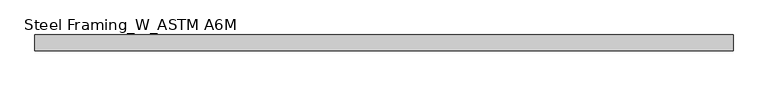
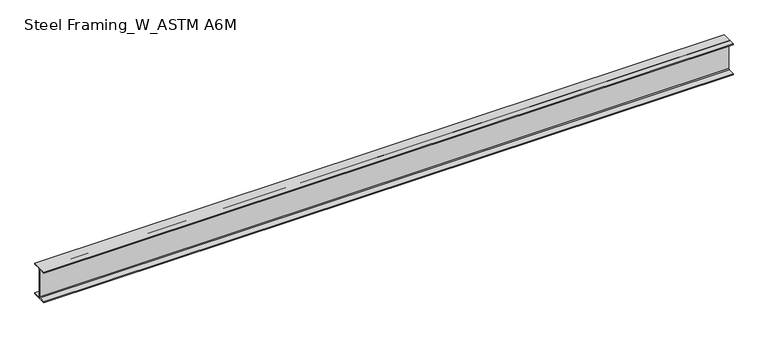
"""IFC4 building model written with IfcOpenShell, lengths in millimetres: beam geometry, Steel Framing_W_ASTM A6M : H_SB_AR_S02_W360x51_RG1."""

import ifcopenshell
import ifcopenshell.guid

model = None  # the IFC model being written
_history = None  # IfcOwnerHistory: only IFC2X3 demands one
_inside = {}  # id of a spatial element -> (the spatial element, [elements in it])
_under = {}  # id of a project, library or spatial element -> (it, [spatial elements below it])
_declared = {}  # id of a project -> (the project, [libraries it declares])
_typed = {}  # id of a type object -> (the type object, [elements of that type])
_made_of = {}  # id of a material, layer set ... -> (it, [elements and type objects made of it])


def new_model(schema):
    """Start an empty IFC model of exactly this schema.

    Asked for "IFC4X3", IfcOpenShell would pick the latest addendum, in which some entities
    have other attributes; the version numbers below select the first issue.
    IFC2X3 requires an IfcOwnerHistory on every rooted entity: one is made here for all.
    """
    global model, _history
    if schema == "IFC4X3":
        model = ifcopenshell.file(schema_version=(4, 3, 0, 0))
    else:
        model = ifcopenshell.file(schema=schema)
    _inside.clear()
    _under.clear()
    _declared.clear()
    _typed.clear()
    _made_of.clear()
    _history = None
    if model.schema == "IFC2X3":
        org = make("IfcOrganization", Name="unknown")
        user = make(
            "IfcPersonAndOrganization",
            ThePerson=make("IfcPerson", FamilyName="unknown"),
            TheOrganization=org,
        )
        app = make(
            "IfcApplication",
            ApplicationDeveloper=org,
            Version="unknown",
            ApplicationFullName="unknown",
            ApplicationIdentifier="unknown",
        )
        _history = make(
            "IfcOwnerHistory",
            OwningUser=user,
            OwningApplication=app,
            ChangeAction="ADDED",
            CreationDate=0,
        )
    return model


def make(cls, **values):
    """One entity of the class cls with the attributes given. An attribute that is None is left unset."""
    return model.create_entity(
        cls, **{name: value for name, value in values.items() if value is not None}
    )


def rooted(cls, **values):
    """An entity with a GlobalId (a new one), such as an element, a storey or a relation."""
    return make(cls, GlobalId=ifcopenshell.guid.new(), OwnerHistory=_history, **values)


def si_unit(unit_type, name, prefix=None):
    """IfcSIUnit, for example si_unit("LENGTHUNIT", "METRE", prefix="MILLI")."""
    return make("IfcSIUnit", UnitType=unit_type, Prefix=prefix, Name=name)


def assignment(units):
    """IfcUnitAssignment: the units of a project."""
    return None if units is None else make("IfcUnitAssignment", Units=units)


def point(xyz):
    """IfcCartesianPoint."""
    return None if xyz is None else make("IfcCartesianPoint", Coordinates=xyz)


def direction(xyz):
    """IfcDirection."""
    return None if xyz is None else make("IfcDirection", DirectionRatios=xyz)


def frame(location, z_axis=None, x_axis=None):
    """IfcAxis2Placement3D, a coordinate frame: its origin and axes. An axis left out is left unset."""
    return make(
        "IfcAxis2Placement3D",
        Location=point(location),
        Axis=direction(z_axis),
        RefDirection=direction(x_axis),
    )


def frame_2d(location, x_axis=None):
    """IfcAxis2Placement2D, a coordinate frame in the plane: its origin and x axis."""
    return make(
        "IfcAxis2Placement2D", Location=point(location), RefDirection=direction(x_axis)
    )


def origin():
    """The frame at (0, 0, 0) with its axes left unset."""
    return frame((0.0, 0.0, 0.0))


def place(relative_to, where):
    """IfcLocalPlacement: puts the frame where relative to a parent placement (None: the world)."""
    return make(
        "IfcLocalPlacement", PlacementRelTo=relative_to, RelativePlacement=where
    )


def context(
    kind, dimensions, precision=None, world=None, true_north=None, identifier=None
):
    """IfcGeometricRepresentationContext, for example the 3D "Model" context."""
    return make(
        "IfcGeometricRepresentationContext",
        ContextIdentifier=identifier,
        ContextType=kind,
        CoordinateSpaceDimension=dimensions,
        Precision=precision,
        WorldCoordinateSystem=world,
        TrueNorth=true_north,
    )


def project(units=None, contexts=None):
    """IfcProject with its units and contexts."""
    return rooted(
        "IfcProject",
        Name="project",
        RepresentationContexts=contexts,
        UnitsInContext=assignment(units),
    )


def spatial(cls, under=None, at=None, **own):
    """A site, building, storey or space (cls), placed at a placement, below another one or the project."""
    s = rooted(cls, ObjectPlacement=at, **own)
    if under is not None:
        _under.setdefault(under.id(), (under, []))[1].append(s)
    return s


def polyline(points):
    """IfcPolyline through the points."""
    return make("IfcPolyline", Points=[point(p) for p in points])


def circle_curve(where, radius):
    """IfcCircle in the frame where."""
    return make("IfcCircle", Position=where, Radius=radius)


def trimmed(basis, trim1, trim2, sense, master):
    """IfcTrimmedCurve: the piece of a basis curve between two trims."""
    return make(
        "IfcTrimmedCurve",
        BasisCurve=basis,
        Trim1=trim1,
        Trim2=trim2,
        SenseAgreement=sense,
        MasterRepresentation=master,
    )


def segment(curve, same_sense, transition):
    """IfcCompositeCurveSegment."""
    return make(
        "IfcCompositeCurveSegment",
        Transition=transition,
        SameSense=same_sense,
        ParentCurve=curve,
    )


def composite_curve(segments, self_intersect=None):
    """IfcCompositeCurve: segments joined end to end."""
    return make("IfcCompositeCurve", Segments=segments, SelfIntersect=self_intersect)


def outline(outer, holes=None, kind="AREA"):
    """IfcArbitraryClosedProfileDef: a profile drawn as a closed curve; with holes, ...WithVoids."""
    if holes is None:
        return make("IfcArbitraryClosedProfileDef", ProfileType=kind, OuterCurve=outer)
    return make(
        "IfcArbitraryProfileDefWithVoids",
        ProfileType=kind,
        OuterCurve=outer,
        InnerCurves=holes,
    )


def extrude(swept, where, along, depth):
    """IfcExtrudedAreaSolid: the profile swept, set in the frame where, extruded along a direction by depth."""
    return make(
        "IfcExtrudedAreaSolid",
        SweptArea=swept,
        Position=where,
        ExtrudedDirection=direction(along),
        Depth=depth,
    )


def shape(context_of_items, identifier, shape_type, items):
    """IfcShapeRepresentation: the items that make up one representation, for example the "Body"."""
    return make(
        "IfcShapeRepresentation",
        ContextOfItems=context_of_items,
        RepresentationIdentifier=identifier,
        RepresentationType=shape_type,
        Items=items,
    )


def source(mapping_origin, context_of_items, identifier, shape_type, items):
    """IfcRepresentationMap: a shape defined once, which mapped items show again and again."""
    return make(
        "IfcRepresentationMap",
        MappingOrigin=mapping_origin,
        MappedRepresentation=shape(context_of_items, identifier, shape_type, items),
    )


def transform(
    local_origin,
    x_axis=None,
    y_axis=None,
    z_axis=None,
    scale=None,
    scale2=None,
    scale3=None,
    uniform=True,
):
    """IfcCartesianTransformationOperator3D, or its non-uniform kind. x_axis, y_axis, z_axis: its Axis1, 2, 3."""
    if uniform:
        return make(
            "IfcCartesianTransformationOperator3D",
            Axis1=direction(x_axis),
            Axis2=direction(y_axis),
            LocalOrigin=point(local_origin),
            Scale=scale,
            Axis3=direction(z_axis),
        )
    return make(
        "IfcCartesianTransformationOperator3DnonUniform",
        Axis1=direction(x_axis),
        Axis2=direction(y_axis),
        LocalOrigin=point(local_origin),
        Scale=scale,
        Axis3=direction(z_axis),
        Scale2=scale2,
        Scale3=scale3,
    )


def mapped(mapping_source, mapping_target):
    """IfcMappedItem: shows the shape of a source again, moved by a transform."""
    return make(
        "IfcMappedItem", MappingSource=mapping_source, MappingTarget=mapping_target
    )


def made_of(thing, what):
    """Note that an element or type object is made of a material, layer set ...; save() writes the relation."""
    if what is not None:
        _made_of.setdefault(what.id(), (what, []))[1].append(thing)
    return thing


def element(
    cls,
    number,
    at=None,
    inside=None,
    cuts=None,
    type_object=None,
    material=None,
    context=None,
    identifier="Body",
    shape_type=None,
    held_by="IfcProductDefinitionShape",
    body=None,
    shapes=None,
    **own,
):
    """One element of the class cls, such as IfcWall. Its Tag is "e" and its number.

    at: its placement. inside: the storey or other place that contains it. cuts: it is an
    opening in that element (IfcRelVoidsElement). A single representation is given by context,
    identifier, shape_type and body (its items); several are given by shapes. held_by: the class
    of the entity that holds the representations. save() writes the other relations.
    """
    e = rooted(cls, Tag="e%d" % number, ObjectPlacement=at, **own)
    if body is not None:
        shapes = [shape(context, identifier, shape_type, body)]
    if shapes is not None:
        e.Representation = make(held_by, Representations=shapes)
    if inside is not None:
        _inside.setdefault(inside.id(), (inside, []))[1].append(e)
    if cuts is not None:
        rooted(
            "IfcRelVoidsElement", RelatingBuildingElement=cuts, RelatedOpeningElement=e
        )
    if type_object is not None:
        _typed.setdefault(type_object.id(), (type_object, []))[1].append(e)
    return made_of(e, material)


def aggregate(whole, parts):
    """IfcRelAggregates: a whole, such as a stair, and the parts it consists of."""
    return rooted("IfcRelAggregates", RelatingObject=whole, RelatedObjects=parts)


def save(model, path):
    """Write the relations noted so far, then the file.

    IfcRelAggregates (storeys below a building ...), IfcRelContainedInSpatialStructure (elements
    in a storey), IfcRelDefinesByType, IfcRelAssociatesMaterial and IfcRelDeclares: one each for
    every whole, place, type object, material and project.
    """
    for whole, parts in _under.values():
        aggregate(whole, parts)
    for where, things in _inside.values():
        rooted(
            "IfcRelContainedInSpatialStructure",
            RelatedElements=things,
            RelatingStructure=where,
        )
    for kind, things in _typed.values():
        rooted("IfcRelDefinesByType", RelatedObjects=things, RelatingType=kind)
    for what, things in _made_of.values():
        rooted("IfcRelAssociatesMaterial", RelatedObjects=things, RelatingMaterial=what)
    for by, libraries in _declared.values():
        rooted("IfcRelDeclares", RelatingContext=by, RelatedDefinitions=libraries)
    model.write(path)


def steel_framing_w_astm_a6m_20e71bf1(model_context):
    return source(origin(), model_context, "Body", "SweptSolid", [
        extrude(outline(composite_curve([segment(polyline([(85.5, -166.4), (85.5, -178.0), (-85.5, -178.0), (-85.5, -166.4), (-13.72, -166.4)]), True, "CONTINUOUS"), segment(trimmed(circle_curve(frame_2d((-13.72, -156.3)), 10.1), [point((-13.72, -166.4))], [point((-3.62, -156.3))], True, "CARTESIAN"), True, "CONTINUOUS"), segment(polyline([(-3.62, -156.3), (-3.62, 156.3)]), True, "CONTINUOUS"), segment(trimmed(circle_curve(frame_2d((-13.72, 156.3)), 10.1), [point((-3.62, 156.3))], [point((-13.72, 166.4))], True, "CARTESIAN"), True, "CONTINUOUS"), segment(polyline([(-13.72, 166.4), (-85.5, 166.4), (-85.5, 178.0), (85.5, 178.0), (85.5, 166.4), (13.72, 166.4)]), True, "CONTINUOUS"), segment(trimmed(circle_curve(frame_2d((13.72, 156.3)), 10.1), [point((13.72, 166.4))], [point((3.62, 156.3))], True, "CARTESIAN"), True, "CONTINUOUS"), segment(polyline([(3.62, 156.3), (3.62, -156.3)]), True, "CONTINUOUS"), segment(trimmed(circle_curve(frame_2d((13.72, -156.3)), 10.1), [point((3.62, -156.3))], [point((13.72, -166.4))], True, "CARTESIAN"), True, "CONTINUOUS"), segment(polyline([(13.72, -166.4), (85.5, -166.4)]), True, "CONTINUOUS")], self_intersect=False)), frame((-3748.7, 0.0, 0.0), z_axis=(1.0, 0.0, 0.0), x_axis=(0.0, 1.0, 0.0)), (0.0, 0.0, 1.0), 7566.7),
    ])


if __name__ == "__main__":
    model = new_model("IFC4")
    model_context = context("Model", 3, world=origin())
    ifc_project = project(units=[si_unit("LENGTHUNIT", "METRE", prefix="MILLI")], contexts=[model_context])
    site = spatial("IfcSite", under=ifc_project)
    building = spatial("IfcBuilding", under=site)
    placement = place(None, origin())
    steel_framing_w_astm_a6m_shape = steel_framing_w_astm_a6m_20e71bf1(model_context)
    element("IfcBeam", 1, ObjectType="Steel Framing_W_ASTM A6M : H_SB_AR_S02_W360x51_RG1", at=placement, inside=building, context=model_context, shape_type="MappedRepresentation", body=[
        mapped(steel_framing_w_astm_a6m_shape, transform((0.0, 0.0, 0.0), x_axis=(1.0, 0.0, 0.0), y_axis=(0.0, 1.0, 0.0), z_axis=(0.0, 0.0, 1.0))),
    ])
    save(model, "model.ifc")

# Revit data of these elements
# Type "Steel Framing_W_ASTM A6M : H_SB_AR_S02_W360x51_RG1"
#   Section Name Key = "W14x34"
#   Width = 17.1 cm
#   Web Thickness = 0.724 cm
#   Web Fillet = 1.01 cm
#   Warping Constant = 287000.0 cm⁶
#   Torsional Moment of Inertia = 23.70 cm⁴
#   Section Area = 64.5 cm²
#   Plastic Modulus weak axis = 174.0 cm³
#   Plastic Modulus strong axis = 895.0 cm³
#   Perimeter = 1.36 m²/m
#   Nominal Weight = 51.00 kgf/m
#   Moment of Inertia weak axis = 970.00 cm⁴
#   Moment of Inertia strong axis = 14200.00 cm⁴
#   Height = 35.6 cm
#   Flange Thickness = 1.16 cm
#   Elastic Modulus weak axis = 113.0 cm³
#   Elastic Modulus strong axis = 796.0 cm³
#   Centroid Vertical = 17.8 cm
#   Centroid Horizontal = 8.55 cm
#   Length [instance default] = 1500 mm
#   Structural Material [instance default] = Steel, 45-345
#   Bolt Spacing = 0
#   Assembly Code = ""
# Element 1 (IfcBeam, "Steel Framing_W_ASTM A6M : H_SB_AR_S02_W360x51_RG1")
#   Materials on its faces: "Steel, 45-345"
# Materials
#   "Steel, 45-345": class "Metal", colour RGB 189 187 185, transparency 0, Description = "Steel 345 MPa", Cost = 0
